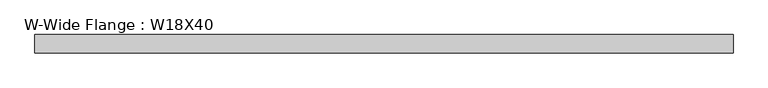
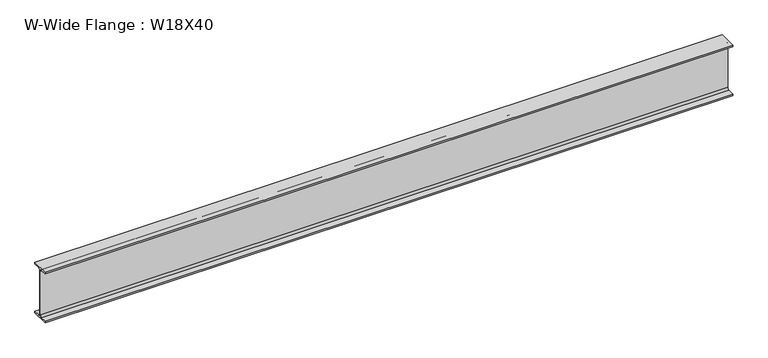
"""IFC4 building model written with IfcOpenShell, lengths in millimetres: beam geometry, W-Wide Flange : W18X40."""

from ifc_helpers import new_model, si_unit, point, frame, frame_2d, origin, place, context, project, spatial, polyline, circle_curve, trimmed, segment, composite_curve, outline, extrude, source, transform, mapped, element, save


def w_wide_flange_w18x40_9f018eca(model_context):
    return source(origin(), model_context, "Body", "SweptSolid", [
        extrude(outline(composite_curve([segment(polyline([(76.454, -213.995), (76.454, -227.33), (-76.454, -227.33), (-76.454, -213.995), (-20.828, -213.995)]), True, "CONTINUOUS"), segment(trimmed(circle_curve(frame_2d((-20.828, -197.1675)), 16.8275), [point((-20.828, -213.995))], [point((-4.0005, -197.1675))], True, "CARTESIAN"), True, "CONTINUOUS"), segment(polyline([(-4.0005, -197.1675), (-4.0005, 197.1675)]), True, "CONTINUOUS"), segment(trimmed(circle_curve(frame_2d((-20.828, 197.1675)), 16.8275), [point((-4.0005, 197.1675))], [point((-20.828, 213.995))], True, "CARTESIAN"), True, "CONTINUOUS"), segment(polyline([(-20.828, 213.995), (-76.454, 213.995), (-76.454, 227.33), (76.454, 227.33), (76.454, 213.995), (20.828, 213.995)]), True, "CONTINUOUS"), segment(trimmed(circle_curve(frame_2d((20.828, 197.1675)), 16.8275), [point((20.828, 213.995))], [point((4.0005, 197.1675))], True, "CARTESIAN"), True, "CONTINUOUS"), segment(polyline([(4.0005, 197.1675), (4.0005, -197.1675)]), True, "CONTINUOUS"), segment(trimmed(circle_curve(frame_2d((20.828, -197.1675)), 16.8275), [point((4.0005, -197.1675))], [point((20.828, -213.995))], True, "CARTESIAN"), True, "CONTINUOUS"), segment(polyline([(20.828, -213.995), (76.454, -213.995)]), True, "CONTINUOUS")], self_intersect=False)), frame((-2907.03, 0.0, 0.0), z_axis=(1.0, 0.0, 0.0), x_axis=(0.0, 1.0, 0.0)), (0.0, 0.0, 1.0), 5870.8925),
    ])


if __name__ == "__main__":
    model = new_model("IFC4")
    model_context = context("Model", 3, world=origin())
    ifc_project = project(units=[si_unit("LENGTHUNIT", "METRE", prefix="MILLI")], contexts=[model_context])
    site = spatial("IfcSite", under=ifc_project)
    building = spatial("IfcBuilding", under=site)
    placement = place(None, origin())
    w_wide_flange_w18x40_shape = w_wide_flange_w18x40_9f018eca(model_context)
    element("IfcBeam", 1, ObjectType="W-Wide Flange : W18X40", at=placement, inside=building, context=model_context, shape_type="MappedRepresentation", body=[
        mapped(w_wide_flange_w18x40_shape, transform((0.0, 0.0, 0.0), x_axis=(1.0, 0.0, 0.0), y_axis=(0.0, 1.0, 0.0), z_axis=(0.0, 0.0, 1.0))),
    ])
    save(model, "model.ifc")

# Revit data of these elements
# Type "W-Wide Flange : W18X40"
#   Assembly Code = "B10"
#   W = 40
#   Length [instance default] = 5' - 0"
#   bf = 0' - 6.02"
#   d = 1' - 5.9"
#   k = 0' - 1 3/16"
#   k2 = 0' - 0.6625"
#   tf = 0' - 0.525"
#   tw = 0' - 0.315"
#   A = 0.0819444 SF
#   Structural Material [instance default] = Steel ASTM A992
# Element 1 (IfcBeam, "W-Wide Flange : W18X40")
#   Materials on its faces: "Steel ASTM A992"
# Materials
#   "Steel ASTM A992": class "Metal", colour RGB 199 199 199, transparency 0, Description = "Structural steel 50ksi", Cost = 0
